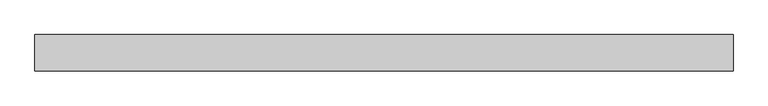
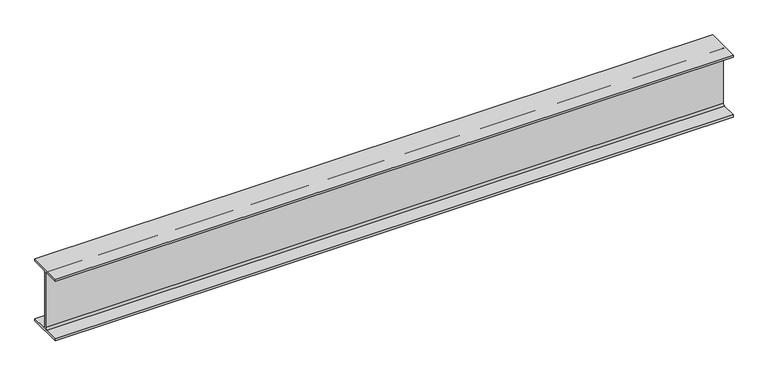
"""IFC4 building model written with IfcOpenShell, lengths in millimetres: beam geometry, Steel Beam_H-KSD3502 : H_SB_ASB_H-250x125x6x9."""

from ifc_helpers import new_model, si_unit, point, frame, frame_2d, origin, place, context, project, spatial, polyline, circle_curve, trimmed, segment, composite_curve, outline, extrude, source, transform, mapped, element, save


def beam_56242eb7(model_context):
    return source(origin(), model_context, "Body", "SweptSolid", [
        extrude(outline(composite_curve([segment(polyline([(82.5, -141.5), (82.5, -151.7), (-82.5, -151.7), (-82.5, -141.5), (-11.9, -141.5)]), True, "CONTINUOUS"), segment(trimmed(circle_curve(frame_2d((-11.9, -132.6)), 8.9), [point((-11.9, -141.5))], [point((-3.0, -132.6))], True, "CARTESIAN"), True, "CONTINUOUS"), segment(polyline([(-3.0, -132.6), (-3.0, 132.6)]), True, "CONTINUOUS"), segment(trimmed(circle_curve(frame_2d((-11.9, 132.6)), 8.9), [point((-3.0, 132.6))], [point((-11.9, 141.5))], True, "CARTESIAN"), True, "CONTINUOUS"), segment(polyline([(-11.9, 141.5), (-82.5, 141.5), (-82.5, 151.7), (82.5, 151.7), (82.5, 141.5), (11.9, 141.5)]), True, "CONTINUOUS"), segment(trimmed(circle_curve(frame_2d((11.9, 132.6)), 8.9), [point((11.9, 141.5))], [point((3.0, 132.6))], True, "CARTESIAN"), True, "CONTINUOUS"), segment(polyline([(3.0, 132.6), (3.0, -132.6)]), True, "CONTINUOUS"), segment(trimmed(circle_curve(frame_2d((11.9, -132.6)), 8.9), [point((3.0, -132.6))], [point((11.9, -141.5))], True, "CARTESIAN"), True, "CONTINUOUS"), segment(polyline([(11.9, -141.5), (82.5, -141.5)]), True, "CONTINUOUS")], self_intersect=False)), frame((-1654.8, 0.0, 0.0), z_axis=(1.0, 0.0, 0.0), x_axis=(0.0, 1.0, 0.0)), (0.0, 0.0, 1.0), 3149.3360727),
    ])


if __name__ == "__main__":
    model = new_model("IFC4")
    model_context = context("Model", 3, world=origin())
    ifc_project = project(units=[si_unit("LENGTHUNIT", "METRE", prefix="MILLI")], contexts=[model_context])
    site = spatial("IfcSite", under=ifc_project)
    building = spatial("IfcBuilding", under=site)
    placement = place(None, origin())
    beam_shape = beam_56242eb7(model_context)
    element("IfcBeam", 1, ObjectType="Steel Beam_H-KSD3502 : H_SB_ASB_H-250x125x6x9", at=placement, inside=building, context=model_context, shape_type="MappedRepresentation", body=[
        mapped(beam_shape, transform((0.0, 0.0, 0.0), x_axis=(1.0, 0.0, 0.0), y_axis=(0.0, 1.0, 0.0), z_axis=(0.0, 0.0, 1.0))),
    ])
    save(model, "model.ifc")

# Revit data of these elements
# Type "Steel Beam_H-KSD3502 : H_SB_ASB_H-250x125x6x9"
#   Width = 12.5 cm
#   Web Thickness = 0.6 cm
#   Web Fillet = 1.2 cm
#   Warping Constant = 42539.8 cm⁶
#   Torsional Moment of Inertia = 7.8102 cm⁴
#   Torsional Modulus = 1.0 cm³
#   Section Area = 37.66 cm²
#   Plastic Modulus weak axis = 73.1 cm³
#   Plastic Modulus strong axis = 366.0 cm³
#   Perimeter = 0.97 m²/m
#   Nominal Weight = 29.60 kgf/m
#   Moment of Inertia weak axis = 294.00 cm⁴
#   Moment of Inertia strong axis = 4050.00 cm⁴
#   Height = 25.0 cm
#   Flange Thickness = 0.9 cm
#   Elastic Modulus weak axis = 47.0 cm³
#   Elastic Modulus strong axis = 324.0 cm³
#   Centroid Vertical = 12.5 cm
#   Centroid Horizontal = 6.25 cm
#   Length [instance default] = 1.5240 m
#   Structural Material [instance default] = Steel, 45-345
#   Assembly Code = ""
# Element 1 (IfcBeam, "Steel Beam_H-KSD3502 : H_SB_ASB_H-250x125x6x9")
#   Structural Material = none
# Materials
#   "Steel, 45-345": class "Metal", colour RGB 189 187 185, transparency 0, Description = "Steel 345 MPa", Cost = 0
